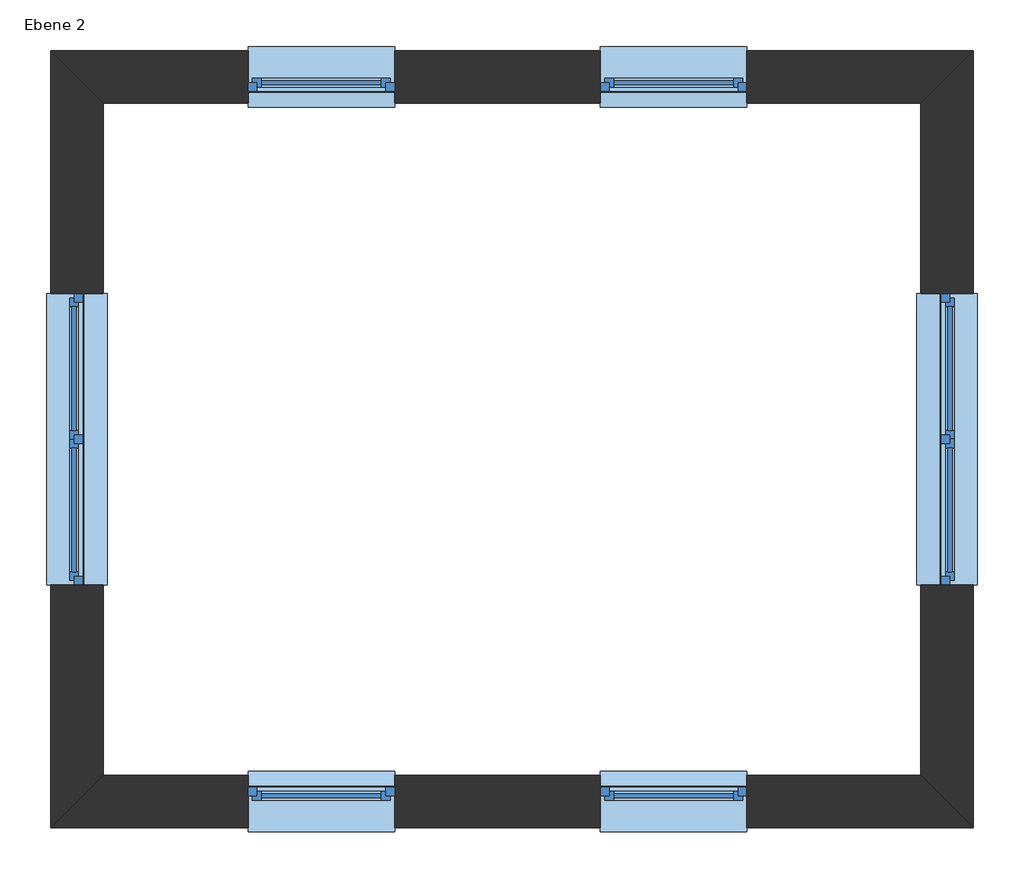
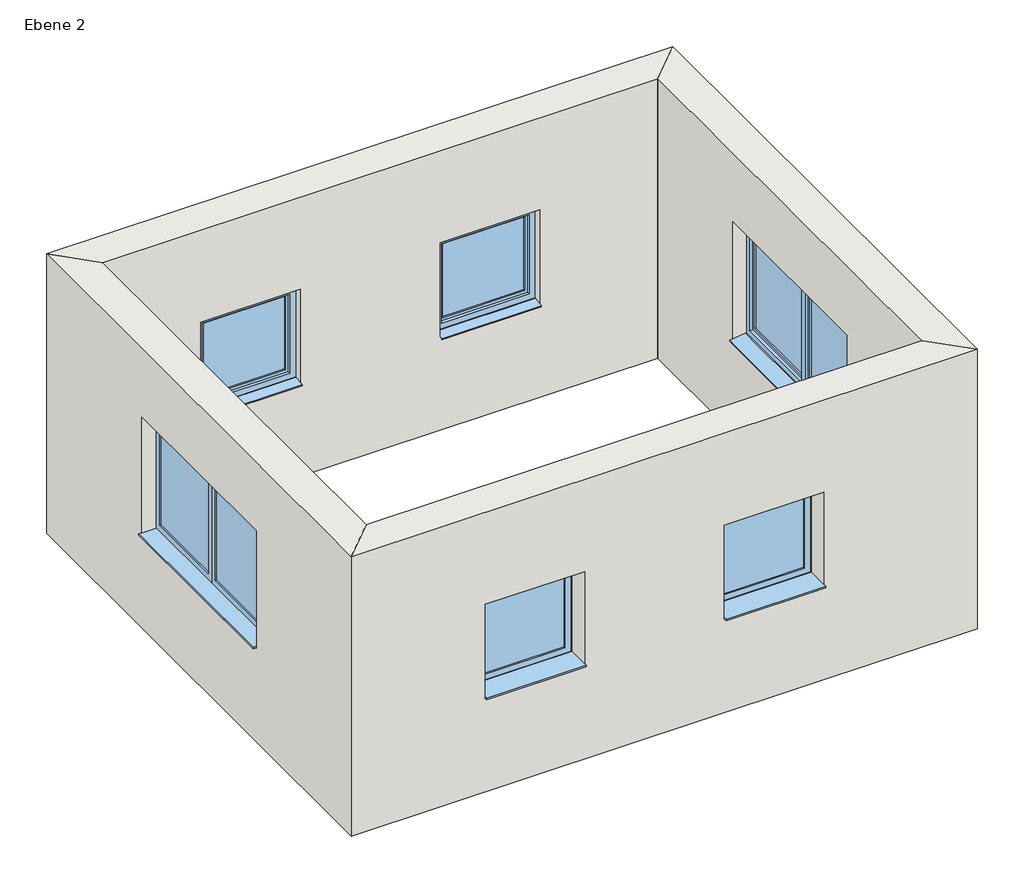
# One storey: 6 windows, 4 walls.
"""IFC4 building model written with IfcOpenShell, lengths in millimetres."""

import ifcopenshell
import ifcopenshell.guid

model = None  # the IFC model being written
_history = None  # IfcOwnerHistory: only IFC2X3 demands one
_inside = {}  # id of a spatial element -> (the spatial element, [elements in it])
_under = {}  # id of a project, library or spatial element -> (it, [spatial elements below it])
_declared = {}  # id of a project -> (the project, [libraries it declares])
_typed = {}  # id of a type object -> (the type object, [elements of that type])
_made_of = {}  # id of a material, layer set ... -> (it, [elements and type objects made of it])


def new_model(schema):
    """Start an empty IFC model of exactly this schema.

    Asked for "IFC4X3", IfcOpenShell would pick the latest addendum, in which some entities
    have other attributes; the version numbers below select the first issue.
    IFC2X3 requires an IfcOwnerHistory on every rooted entity: one is made here for all.
    """
    global model, _history
    if schema == "IFC4X3":
        model = ifcopenshell.file(schema_version=(4, 3, 0, 0))
    else:
        model = ifcopenshell.file(schema=schema)
    _inside.clear()
    _under.clear()
    _declared.clear()
    _typed.clear()
    _made_of.clear()
    _history = None
    if model.schema == "IFC2X3":
        org = make("IfcOrganization", Name="unknown")
        user = make(
            "IfcPersonAndOrganization",
            ThePerson=make("IfcPerson", FamilyName="unknown"),
            TheOrganization=org,
        )
        app = make(
            "IfcApplication",
            ApplicationDeveloper=org,
            Version="unknown",
            ApplicationFullName="unknown",
            ApplicationIdentifier="unknown",
        )
        _history = make(
            "IfcOwnerHistory",
            OwningUser=user,
            OwningApplication=app,
            ChangeAction="ADDED",
            CreationDate=0,
        )
    return model


def make(cls, **values):
    """One entity of the class cls with the attributes given. An attribute that is None is left unset."""
    return model.create_entity(
        cls, **{name: value for name, value in values.items() if value is not None}
    )


def rooted(cls, **values):
    """An entity with a GlobalId (a new one), such as an element, a storey or a relation."""
    return make(cls, GlobalId=ifcopenshell.guid.new(), OwnerHistory=_history, **values)


def si_unit(unit_type, name, prefix=None):
    """IfcSIUnit, for example si_unit("LENGTHUNIT", "METRE", prefix="MILLI")."""
    return make("IfcSIUnit", UnitType=unit_type, Prefix=prefix, Name=name)


def assignment(units):
    """IfcUnitAssignment: the units of a project."""
    return None if units is None else make("IfcUnitAssignment", Units=units)


def point(xyz):
    """IfcCartesianPoint."""
    return None if xyz is None else make("IfcCartesianPoint", Coordinates=xyz)


def direction(xyz):
    """IfcDirection."""
    return None if xyz is None else make("IfcDirection", DirectionRatios=xyz)


def frame(location, z_axis=None, x_axis=None):
    """IfcAxis2Placement3D, a coordinate frame: its origin and axes. An axis left out is left unset."""
    return make(
        "IfcAxis2Placement3D",
        Location=point(location),
        Axis=direction(z_axis),
        RefDirection=direction(x_axis),
    )


def origin():
    """The frame at (0, 0, 0) with its axes left unset."""
    return frame((0.0, 0.0, 0.0))


def place(relative_to, where):
    """IfcLocalPlacement: puts the frame where relative to a parent placement (None: the world)."""
    return make(
        "IfcLocalPlacement", PlacementRelTo=relative_to, RelativePlacement=where
    )


def context(
    kind, dimensions, precision=None, world=None, true_north=None, identifier=None
):
    """IfcGeometricRepresentationContext, for example the 3D "Model" context."""
    return make(
        "IfcGeometricRepresentationContext",
        ContextIdentifier=identifier,
        ContextType=kind,
        CoordinateSpaceDimension=dimensions,
        Precision=precision,
        WorldCoordinateSystem=world,
        TrueNorth=true_north,
    )


def project(units=None, contexts=None):
    """IfcProject with its units and contexts."""
    return rooted(
        "IfcProject",
        Name="project",
        RepresentationContexts=contexts,
        UnitsInContext=assignment(units),
    )


def spatial(cls, under=None, at=None, **own):
    """A site, building, storey or space (cls), placed at a placement, below another one or the project."""
    s = rooted(cls, ObjectPlacement=at, **own)
    if under is not None:
        _under.setdefault(under.id(), (under, []))[1].append(s)
    return s


def polyline(points):
    """IfcPolyline through the points."""
    return make("IfcPolyline", Points=[point(p) for p in points])


def outline(outer, holes=None, kind="AREA"):
    """IfcArbitraryClosedProfileDef: a profile drawn as a closed curve; with holes, ...WithVoids."""
    if holes is None:
        return make("IfcArbitraryClosedProfileDef", ProfileType=kind, OuterCurve=outer)
    return make(
        "IfcArbitraryProfileDefWithVoids",
        ProfileType=kind,
        OuterCurve=outer,
        InnerCurves=holes,
    )


def extrude(swept, where, along, depth):
    """IfcExtrudedAreaSolid: the profile swept, set in the frame where, extruded along a direction by depth."""
    return make(
        "IfcExtrudedAreaSolid",
        SweptArea=swept,
        Position=where,
        ExtrudedDirection=direction(along),
        Depth=depth,
    )


def faces_of(points, faces, orient=None, outer=None):
    """IfcFace entities. A face is a list of loops; a loop is a list of indices into points, from 0.

    orient and outer hold one flag for each loop. By default every Orientation is true, the
    first loop of a face is its IfcFaceOuterBound and the others are IfcFaceBound.
    """
    made = []
    for i, loops in enumerate(faces):
        bounds = []
        for j, loop in enumerate(loops):
            is_outer = j == 0 if outer is None else outer[i][j]
            bounds.append(
                make(
                    "IfcFaceOuterBound" if is_outer else "IfcFaceBound",
                    Bound=make("IfcPolyLoop", Polygon=[points[k] for k in loop]),
                    Orientation=True if orient is None else orient[i][j],
                )
            )
        made.append(make("IfcFace", Bounds=bounds))
    return made


def faceted_brep(points, faces, orient=None, outer=None, voids=None):
    """IfcFacetedBrep: a solid bounded by flat faces; with voids (closed shells), ...WithVoids."""
    shared = [point(p) for p in points]
    hull = make("IfcClosedShell", CfsFaces=faces_of(shared, faces, orient, outer))
    if voids is None:
        return make("IfcFacetedBrep", Outer=hull)
    return make(
        "IfcFacetedBrepWithVoids",
        Outer=hull,
        Voids=[
            make(cls, CfsFaces=faces_of(shared, fs, o, b)) for cls, fs, o, b in voids
        ],
    )


def shape(context_of_items, identifier, shape_type, items):
    """IfcShapeRepresentation: the items that make up one representation, for example the "Body"."""
    return make(
        "IfcShapeRepresentation",
        ContextOfItems=context_of_items,
        RepresentationIdentifier=identifier,
        RepresentationType=shape_type,
        Items=items,
    )


def source(mapping_origin, context_of_items, identifier, shape_type, items):
    """IfcRepresentationMap: a shape defined once, which mapped items show again and again."""
    return make(
        "IfcRepresentationMap",
        MappingOrigin=mapping_origin,
        MappedRepresentation=shape(context_of_items, identifier, shape_type, items),
    )


def transform(
    local_origin,
    x_axis=None,
    y_axis=None,
    z_axis=None,
    scale=None,
    scale2=None,
    scale3=None,
    uniform=True,
):
    """IfcCartesianTransformationOperator3D, or its non-uniform kind. x_axis, y_axis, z_axis: its Axis1, 2, 3."""
    if uniform:
        return make(
            "IfcCartesianTransformationOperator3D",
            Axis1=direction(x_axis),
            Axis2=direction(y_axis),
            LocalOrigin=point(local_origin),
            Scale=scale,
            Axis3=direction(z_axis),
        )
    return make(
        "IfcCartesianTransformationOperator3DnonUniform",
        Axis1=direction(x_axis),
        Axis2=direction(y_axis),
        LocalOrigin=point(local_origin),
        Scale=scale,
        Axis3=direction(z_axis),
        Scale2=scale2,
        Scale3=scale3,
    )


def mapped(mapping_source, mapping_target):
    """IfcMappedItem: shows the shape of a source again, moved by a transform."""
    return make(
        "IfcMappedItem", MappingSource=mapping_source, MappingTarget=mapping_target
    )


def made_of(thing, what):
    """Note that an element or type object is made of a material, layer set ...; save() writes the relation."""
    if what is not None:
        _made_of.setdefault(what.id(), (what, []))[1].append(thing)
    return thing


def element(
    cls,
    number,
    at=None,
    inside=None,
    cuts=None,
    type_object=None,
    material=None,
    context=None,
    identifier="Body",
    shape_type=None,
    held_by="IfcProductDefinitionShape",
    body=None,
    shapes=None,
    **own,
):
    """One element of the class cls, such as IfcWall. Its Tag is "e" and its number.

    at: its placement. inside: the storey or other place that contains it. cuts: it is an
    opening in that element (IfcRelVoidsElement). A single representation is given by context,
    identifier, shape_type and body (its items); several are given by shapes. held_by: the class
    of the entity that holds the representations. save() writes the other relations.
    """
    e = rooted(cls, Tag="e%d" % number, ObjectPlacement=at, **own)
    if body is not None:
        shapes = [shape(context, identifier, shape_type, body)]
    if shapes is not None:
        e.Representation = make(held_by, Representations=shapes)
    if inside is not None:
        _inside.setdefault(inside.id(), (inside, []))[1].append(e)
    if cuts is not None:
        rooted(
            "IfcRelVoidsElement", RelatingBuildingElement=cuts, RelatedOpeningElement=e
        )
    if type_object is not None:
        _typed.setdefault(type_object.id(), (type_object, []))[1].append(e)
    return made_of(e, material)


def aggregate(whole, parts):
    """IfcRelAggregates: a whole, such as a stair, and the parts it consists of."""
    return rooted("IfcRelAggregates", RelatingObject=whole, RelatedObjects=parts)


def save(model, path):
    """Write the relations noted so far, then the file.

    IfcRelAggregates (storeys below a building ...), IfcRelContainedInSpatialStructure (elements
    in a storey), IfcRelDefinesByType, IfcRelAssociatesMaterial and IfcRelDeclares: one each for
    every whole, place, type object, material and project.
    """
    for whole, parts in _under.values():
        aggregate(whole, parts)
    for where, things in _inside.values():
        rooted(
            "IfcRelContainedInSpatialStructure",
            RelatedElements=things,
            RelatingStructure=where,
        )
    for kind, things in _typed.values():
        rooted("IfcRelDefinesByType", RelatedObjects=things, RelatingType=kind)
    for what, things in _made_of.values():
        rooted("IfcRelAssociatesMaterial", RelatedObjects=things, RelatingMaterial=what)
    for by, libraries in _declared.values():
        rooted("IfcRelDeclares", RelatingContext=by, RelatedDefinitions=libraries)
    model.write(path)


def fenster_1_flg_variabel_fenster_1_flg_variabel_3_8a378bad(model_context):
    return source(origin(), model_context, "Body", "SolidModel", [
        extrude(outline(polyline([(2010.0, 505.0), (2010.0, -505.0), (1000.0, -505.0), (1000.0, 505.0), (2010.0, 505.0)]), holes=[polyline([(1930.0, 445.0), (1080.0, 445.0), (1080.0, -445.0), (1930.0, -445.0), (1930.0, 445.0)])]), frame((0.0, 40.0, 0.0), z_axis=(0.0, 1.0, 0.0), x_axis=(0.0, 0.0, 1.0)), (0.0, 0.0, 1.0), 60.0),
        faceted_brep([(475.0, 40.0, 1960.0), (475.0, 10.0, 1960.0), (475.0, 10.0, 1050.0), (475.0, 40.0, 1050.0), (-475.0, 10.0, 1960.0), (-475.0, 10.0, 1050.0), (415.0, 10.0, 1110.0), (-415.0, 10.0, 1110.0), (-415.0, 10.0, 1900.0), (415.0, 10.0, 1900.0), (-475.0, 40.0, 1050.0), (-475.0, 40.0, 1960.0), (445.0, 40.0, 1930.0), (-445.0, 40.0, 1930.0), (-445.0, 40.0, 1080.0), (445.0, 40.0, 1080.0), (445.0, 70.0, 1930.0), (445.0, 70.0, 1080.0), (-445.0, 70.0, 1080.0), (-445.0, 70.0, 1930.0), (415.0, 70.0, 1900.0), (-415.0, 70.0, 1900.0), (-415.0, 70.0, 1110.0), (415.0, 70.0, 1110.0)], [[[0, 1, 2, 3]], [[1, 4, 5, 2], [6, 7, 8, 9]], [[3, 2, 5, 10]], [[3, 10, 11, 0], [12, 13, 14, 15]], [[16, 12, 15, 17]], [[17, 15, 14, 18]], [[17, 18, 19, 16], [20, 21, 22, 23]], [[9, 20, 23, 6]], [[6, 23, 22, 7]], [[10, 5, 4, 11]], [[18, 14, 13, 19]], [[7, 22, 21, 8]], [[11, 4, 1, 0]], [[19, 13, 12, 16]], [[8, 21, 20, 9]]]),
        extrude(outline(polyline([(-505.0, -210.0), (-505.0, 40.0), (505.0, 40.0), (505.0, -210.0), (-505.0, -210.0)])), frame((0.0, 0.0, 1005.0), z_axis=(0.0, 0.0, 1.0), x_axis=(1.0, 0.0, 0.0)), (0.0, 0.0, 1.0), 15.0),
        extrude(outline(polyline([(110.0221543, 1020.0), (210.0, 1000.0), (210.0, 990.0), (208.0, 990.0), (208.0, 998.3604634), (109.8240723, 1018.0), (100.0, 1018.0), (100.0, 1020.0), (110.0221543, 1020.0)])), frame((-505.0, 0.0, 0.0), z_axis=(1.0, 0.0, 0.0), x_axis=(0.0, 1.0, 0.0)), (0.0, 0.0, 1.0), 1010.0),
        extrude(outline(polyline([(415.0, 25.0), (-415.0, 25.0), (-415.0, 55.0), (415.0, 55.0), (415.0, 25.0)])), frame((0.0, 0.0, 1110.0), z_axis=(0.0, 0.0, 1.0), x_axis=(1.0, 0.0, 0.0)), (0.0, 0.0, 1.0), 790.0),
    ])


def fenster_2_flg_variabel_fenster_2_flg_variabel_3_03287464(model_context):
    return source(origin(), model_context, "Body", "SolidModel", [
        extrude(outline(polyline([(60.0, -5.0), (915.0, -5.0), (915.0, -35.0), (60.0, -35.0), (60.0, -5.0)])), frame((0.0, 0.0, 1110.0), z_axis=(0.0, 0.0, 1.0), x_axis=(1.0, 0.0, 0.0)), (0.0, 0.0, 1.0), 1040.0),
        extrude(outline(polyline([(-915.0, -5.0), (-60.0, -5.0), (-60.0, -35.0), (-915.0, -35.0), (-915.0, -5.0)])), frame((0.0, 0.0, 1110.0), z_axis=(0.0, 0.0, 1.0), x_axis=(1.0, 0.0, 0.0)), (0.0, 0.0, 1.0), 1040.0),
        extrude(outline(polyline([(-1005.0, -210.0), (-1005.0, -20.0), (1005.0, -20.0), (1005.0, -210.0), (-1005.0, -210.0)])), frame((0.0, 0.0, 1005.0), z_axis=(0.0, 0.0, 1.0), x_axis=(1.0, 0.0, 0.0)), (0.0, 0.0, 1.0), 15.0),
        extrude(outline(polyline([(50.0221543, 1020.0), (210.0, 1000.0), (210.0, 990.0), (208.0, 990.0), (208.0, 998.3604634), (49.8240723, 1018.0), (40.0, 1018.0), (40.0, 1020.0), (50.0221543, 1020.0)])), frame((-1005.0, 0.0, 0.0), z_axis=(1.0, 0.0, 0.0), x_axis=(0.0, 1.0, 0.0)), (0.0, 0.0, 1.0), 2010.0),
        extrude(outline(polyline([(30.0, -20.0), (-30.0, -20.0), (-30.0, 40.0), (30.0, 40.0), (30.0, -20.0)])), frame((0.0, 0.0, 1080.0), z_axis=(0.0, 0.0, 1.0), x_axis=(1.0, 0.0, 0.0)), (0.0, 0.0, 1.0), 1100.0),
        extrude(outline(polyline([(2260.0, -1005.0), (1000.0, -1005.0), (1000.0, 1005.0), (2260.0, 1005.0), (2260.0, -1005.0)]), holes=[polyline([(2180.0, -945.0), (2180.0, 945.0), (1080.0, 945.0), (1080.0, -945.0), (2180.0, -945.0)])]), frame((0.0, -20.0, 0.0), z_axis=(0.0, 1.0, 0.0), x_axis=(0.0, 0.0, 1.0)), (0.0, 0.0, 1.0), 60.0),
        faceted_brep([(-945.0, -20.0, 1080.0), (-945.0, 10.0, 1080.0), (-30.0, 10.0, 1080.0), (-30.0, -20.0, 1080.0), (-30.0, 10.0, 2180.0), (-30.0, -20.0, 2180.0), (-945.0, 10.0, 2180.0), (-60.0, 10.0, 2150.0), (-915.0, 10.0, 2150.0), (-915.0, 10.0, 1110.0), (-60.0, 10.0, 1110.0), (0.0, -20.0, 1050.0), (-975.0, -20.0, 1050.0), (-975.0, -20.0, 2210.0), (0.0, -20.0, 2210.0), (-945.0, -20.0, 2180.0), (-975.0, -50.0, 1050.0), (0.0, -50.0, 1050.0), (0.0, -50.0, 2210.0), (-975.0, -50.0, 2210.0), (-60.0, -50.0, 1110.0), (-915.0, -50.0, 1110.0), (-915.0, -50.0, 2150.0), (-60.0, -50.0, 2150.0)], [[[0, 1, 2, 3]], [[3, 2, 4, 5]], [[2, 1, 6, 4], [7, 8, 9, 10]], [[11, 12, 13, 14], [5, 15, 0, 3]], [[16, 12, 11, 17]], [[17, 11, 14, 18]], [[18, 19, 16, 17], [20, 21, 22, 23]], [[9, 21, 20, 10]], [[10, 20, 23, 7]], [[15, 6, 1, 0]], [[19, 13, 12, 16]], [[8, 22, 21, 9]], [[5, 4, 6, 15]], [[18, 14, 13, 19]], [[7, 23, 22, 8]]]),
        faceted_brep([(30.0, -20.0, 1080.0), (30.0, 10.0, 1080.0), (945.0, 10.0, 1080.0), (945.0, -20.0, 1080.0), (945.0, 10.0, 2180.0), (945.0, -20.0, 2180.0), (30.0, 10.0, 2180.0), (915.0, 10.0, 2150.0), (60.0, 10.0, 2150.0), (60.0, 10.0, 1110.0), (915.0, 10.0, 1110.0), (975.0, -20.0, 1050.0), (0.0, -20.0, 1050.0), (0.0, -20.0, 2210.0), (975.0, -20.0, 2210.0), (30.0, -20.0, 2180.0), (0.0, -50.0, 1050.0), (975.0, -50.0, 1050.0), (975.0, -50.0, 2210.0), (0.0, -50.0, 2210.0), (915.0, -50.0, 1110.0), (60.0, -50.0, 1110.0), (60.0, -50.0, 2150.0), (915.0, -50.0, 2150.0)], [[[0, 1, 2, 3]], [[3, 2, 4, 5]], [[2, 1, 6, 4], [7, 8, 9, 10]], [[11, 12, 13, 14], [5, 15, 0, 3]], [[16, 12, 11, 17]], [[17, 11, 14, 18]], [[18, 19, 16, 17], [20, 21, 22, 23]], [[9, 21, 20, 10]], [[10, 20, 23, 7]], [[15, 6, 1, 0]], [[19, 13, 12, 16]], [[8, 22, 21, 9]], [[5, 4, 6, 15]], [[18, 14, 13, 19]], [[7, 23, 22, 8]]]),
    ])


model = new_model("IFC4")

# Units and contexts
model_context = context("Model", 3, world=origin())
ifc_project = project(units=[si_unit("LENGTHUNIT", "METRE", prefix="MILLI")], contexts=[model_context])

# Site, building, storey
site = spatial("IfcSite", under=ifc_project)
building = spatial("IfcBuilding", under=site)
storey = spatial("IfcBuildingStorey", under=building, Name="Ebene 2", Elevation=6000.0)

# Walls
placement = place(None, origin())
element("IfcWall", 1, ObjectType="MW 24.0 WD 12.0", at=placement, inside=storey, context=model_context, shape_type="Brep", body=[
    faceted_brep([(-6003.5987005, 5004.2257101, 6000.0), (-363.5987005, 5004.2257101, 6000.0), (-363.5987005, 5004.2257101, 9000.0), (-6003.5987005, 5004.2257101, 9000.0), (-1563.5987005, 5004.2257101, 7000.0), (-2573.5987005, 5004.2257101, 7000.0), (-2573.5987005, 5004.2257101, 8010.0), (-1563.5987005, 5004.2257101, 8010.0), (-3993.5987005, 5004.2257101, 7000.0), (-5003.5987005, 5004.2257101, 7000.0), (-5003.5987005, 5004.2257101, 8010.0), (-3993.5987005, 5004.2257101, 8010.0), (-6363.5987005, 5364.2257101, 6000.0), (-6363.5987005, 5364.2257101, 9000.0), (-3.5987005, 5364.2257101, 9000.0), (-3.5987005, 5364.2257101, 6000.0), (-1563.5987005, 5364.2257101, 7000.0), (-1563.5987005, 5364.2257101, 8010.0), (-2573.5987005, 5364.2257101, 8010.0), (-2573.5987005, 5364.2257101, 7000.0), (-3993.5987005, 5364.2257101, 7000.0), (-3993.5987005, 5364.2257101, 8010.0), (-5003.5987005, 5364.2257101, 8010.0), (-5003.5987005, 5364.2257101, 7000.0)], [[[0, 1, 2, 3], [4, 5, 6, 7], [8, 9, 10, 11]], [[12, 13, 14, 15], [16, 17, 18, 19], [20, 21, 22, 23]], [[1, 0, 12, 15]], [[3, 2, 14, 13]], [[2, 1, 15, 14]], [[0, 3, 13, 12]], [[17, 16, 4, 7]], [[18, 17, 7, 6]], [[19, 18, 6, 5]], [[16, 19, 5, 4]], [[21, 20, 8, 11]], [[22, 21, 11, 10]], [[23, 22, 10, 9]], [[20, 23, 9, 8]]]),
])
element("IfcWall", 2, ObjectType="MW 24.0 WD 12.0", at=placement, inside=storey, context=model_context, shape_type="Brep", body=[
    faceted_brep([(-363.5987005, 5004.2257101, 6000.0), (-363.5987005, 364.2257101, 6000.0), (-363.5987005, 364.2257101, 9000.0), (-363.5987005, 5004.2257101, 9000.0), (-363.5987005, 1679.2257101, 7000.0), (-363.5987005, 3689.2257101, 7000.0), (-363.5987005, 3689.2257101, 8260.0), (-363.5987005, 1679.2257101, 8260.0), (-3.5987005, 5364.2257101, 6000.0), (-3.5987005, 5364.2257101, 9000.0), (-3.5987005, 4.2257101, 9000.0), (-3.5987005, 4.2257101, 6000.0), (-3.5987005, 1679.2257101, 7000.0), (-3.5987005, 1679.2257101, 8260.0), (-3.5987005, 3689.2257101, 8260.0), (-3.5987005, 3689.2257101, 7000.0)], [[[0, 1, 2, 3], [4, 5, 6, 7]], [[8, 9, 10, 11], [12, 13, 14, 15]], [[1, 0, 8, 11]], [[3, 2, 10, 9]], [[0, 3, 9, 8]], [[2, 1, 11, 10]], [[13, 12, 4, 7]], [[14, 13, 7, 6]], [[15, 14, 6, 5]], [[12, 15, 5, 4]]]),
])
element("IfcWall", 3, ObjectType="MW 24.0 WD 12.0", at=placement, inside=storey, context=model_context, shape_type="Brep", body=[
    faceted_brep([(-363.5987005, 364.2257101, 6000.0), (-6003.5987005, 364.2257101, 6000.0), (-6003.5987005, 364.2257101, 9000.0), (-363.5987005, 364.2257101, 9000.0), (-2573.5987005, 364.2257101, 7000.0), (-1563.5987005, 364.2257101, 7000.0), (-1563.5987005, 364.2257101, 8010.0), (-2573.5987005, 364.2257101, 8010.0), (-5003.5987005, 364.2257101, 7000.0), (-3993.5987005, 364.2257101, 7000.0), (-3993.5987005, 364.2257101, 8010.0), (-5003.5987005, 364.2257101, 8010.0), (-3.5987005, 4.2257101, 6000.0), (-3.5987005, 4.2257101, 9000.0), (-6363.5987005, 4.2257101, 9000.0), (-6363.5987005, 4.2257101, 6000.0), (-2573.5987005, 4.2257101, 7000.0), (-2573.5987005, 4.2257101, 8010.0), (-1563.5987005, 4.2257101, 8010.0), (-1563.5987005, 4.2257101, 7000.0), (-5003.5987005, 4.2257101, 7000.0), (-5003.5987005, 4.2257101, 8010.0), (-3993.5987005, 4.2257101, 8010.0), (-3993.5987005, 4.2257101, 7000.0)], [[[0, 1, 2, 3], [4, 5, 6, 7], [8, 9, 10, 11]], [[12, 13, 14, 15], [16, 17, 18, 19], [20, 21, 22, 23]], [[1, 0, 12, 15]], [[3, 2, 14, 13]], [[0, 3, 13, 12]], [[2, 1, 15, 14]], [[17, 16, 4, 7]], [[18, 17, 7, 6]], [[19, 18, 6, 5]], [[16, 19, 5, 4]], [[21, 20, 8, 11]], [[22, 21, 11, 10]], [[23, 22, 10, 9]], [[20, 23, 9, 8]]]),
])
element("IfcWall", 4, ObjectType="MW 24.0 WD 12.0", at=placement, inside=storey, context=model_context, shape_type="Brep", body=[
    faceted_brep([(-6003.5987005, 364.2257101, 6000.0), (-6003.5987005, 5004.2257101, 6000.0), (-6003.5987005, 5004.2257101, 9000.0), (-6003.5987005, 364.2257101, 9000.0), (-6003.5987005, 3689.2257101, 7000.0), (-6003.5987005, 1679.2257101, 7000.0), (-6003.5987005, 1679.2257101, 8260.0), (-6003.5987005, 3689.2257101, 8260.0), (-6363.5987005, 4.2257101, 6000.0), (-6363.5987005, 4.2257101, 9000.0), (-6363.5987005, 5364.2257101, 9000.0), (-6363.5987005, 5364.2257101, 6000.0), (-6363.5987005, 3689.2257101, 7000.0), (-6363.5987005, 3689.2257101, 8260.0), (-6363.5987005, 1679.2257101, 8260.0), (-6363.5987005, 1679.2257101, 7000.0)], [[[0, 1, 2, 3], [4, 5, 6, 7]], [[8, 9, 10, 11], [12, 13, 14, 15]], [[1, 0, 8, 11]], [[3, 2, 10, 9]], [[2, 1, 11, 10]], [[0, 3, 9, 8]], [[13, 12, 4, 7]], [[14, 13, 7, 6]], [[15, 14, 6, 5]], [[12, 15, 5, 4]]]),
])

# Windows
fenster_1_flg_variabel_fenster_1_flg_variabel_3_shape = fenster_1_flg_variabel_fenster_1_flg_variabel_3_8a378bad(model_context)
element("IfcWindow", 5, ObjectType="Fenster 1-flg - Variabel : Fenster 1-flg - Variabel 3", at=placement, inside=storey, context=model_context, shape_type="MappedRepresentation", body=[
    mapped(fenster_1_flg_variabel_fenster_1_flg_variabel_3_shape, transform((-2068.5987005, 184.2257101, 6000.0), x_axis=(1.0, 0.0, 0.0), y_axis=(0.0, 1.0, 0.0), z_axis=(0.0, 0.0, 1.0))),
])
element("IfcWindow", 6, ObjectType="Fenster 1-flg - Variabel : Fenster 1-flg - Variabel 3", at=placement, inside=storey, context=model_context, shape_type="MappedRepresentation", body=[
    mapped(fenster_1_flg_variabel_fenster_1_flg_variabel_3_shape, transform((-4498.5987005, 184.2257101, 6000.0), x_axis=(1.0, 0.0, 0.0), y_axis=(0.0, 1.0, 0.0), z_axis=(0.0, 0.0, 1.0))),
])
element("IfcWindow", 7, ObjectType="Fenster 1-flg - Variabel : Fenster 1-flg - Variabel 3", at=placement, inside=storey, context=model_context, shape_type="MappedRepresentation", body=[
    mapped(fenster_1_flg_variabel_fenster_1_flg_variabel_3_shape, transform((-2068.5987005, 5184.2257101, 6000.0), x_axis=(-1.0, 0.0, 0.0), y_axis=(0.0, -1.0, 0.0), z_axis=(0.0, 0.0, 1.0))),
])
element("IfcWindow", 8, ObjectType="Fenster 1-flg - Variabel : Fenster 1-flg - Variabel 3", at=placement, inside=storey, context=model_context, shape_type="MappedRepresentation", body=[
    mapped(fenster_1_flg_variabel_fenster_1_flg_variabel_3_shape, transform((-4498.5987005, 5184.2257101, 6000.0), x_axis=(-1.0, 0.0, 0.0), y_axis=(0.0, -1.0, 0.0), z_axis=(0.0, 0.0, 1.0))),
])
fenster_2_flg_variabel_fenster_2_flg_variabel_3_shape = fenster_2_flg_variabel_fenster_2_flg_variabel_3_03287464(model_context)
element("IfcWindow", 9, ObjectType="Fenster 2-flg - Variabel : Fenster 2-flg - Variabel 3", at=placement, inside=storey, context=model_context, shape_type="MappedRepresentation", body=[
    mapped(fenster_2_flg_variabel_fenster_2_flg_variabel_3_shape, transform((-183.5987005, 2684.2257101, 6000.0), x_axis=(0.0, 1.0, 0.0), y_axis=(-1.0, 0.0, 0.0), z_axis=(0.0, 0.0, 1.0))),
])
element("IfcWindow", 10, ObjectType="Fenster 2-flg - Variabel : Fenster 2-flg - Variabel 3", at=placement, inside=storey, context=model_context, shape_type="MappedRepresentation", body=[
    mapped(fenster_2_flg_variabel_fenster_2_flg_variabel_3_shape, transform((-6183.5987005, 2684.2257101, 6000.0), x_axis=(0.0, -1.0, 0.0), y_axis=(1.0, 0.0, 0.0), z_axis=(0.0, 0.0, 1.0))),
])

save(model, "model.ifc")

# Revit data of these elements
# Type "MW 24.0 WD 12.0"
#   Type Comments = "Mehrschaliges Mauerwerk"
#   Description = "Mauerwerk 24.0 cm, Wärmedämmung 12.0 cm"
#   Layers, outside or top first: 0.120 m "Wärmedämmung - hart" (function 3); 0.240 m "Mauerwerk - Ziegel, verputzt" (function 1)
# Type "Fenster 1-flg - Variabel : Fenster 1-flg - Variabel 3"
#   Type Mark = "52"
#   Operation = "SinglePanel"
#   Construction Type Id = "GSP4R"
#   Keynote = "16.05.01"
#   Analytic Construction = "1/8 Zoll Pilkington-Verglasung einfach"
#   Cost = 78.2
#   Visual Light Transmittance = 0.9
#   Höhe oberer  Rahmen = 0.080 m
#   Solar Heat Gain Coefficient = 0.86
#   Tiefe Flügel = 0.060 m
#   Rough Width [instance default] = 1.010 m
#   Rough Height [instance default] = 1.010 m
#   Rahmenhöhe unten = 0.080 m
#   Heat Transfer Coefficient (U) = 6.7069 W/(m²·K)
#   Rahmentiefe = 0.060 m
#   Rahmenbreite = 0.060 m
#   Height [instance default] = 1.010 m
#   Flügelbreite = 0.060 m
#   Einbautiefe (von außen) [instance default] = 0.080 m
#   Width [instance default] = 1.010 m
#   Define Thermal Properties by = 1
#   Öffnungsrichtung oben [instance default] = yes
#   Öffnungsrichtung in Draufsicht anzeigen [instance default] = no
#   Klappflügel [instance default] = no
#   Drehflügel 1 [instance default] = yes
#   Fensterflügel [instance default] = none
#   Innere Fensterbank [instance default] = none
#   Glas [instance default] = none
#   Bild [instance default] = none
#   Äußere Fensterbank [instance default] = none
#   Wall Closure = (empty or 0)
# Type "Fenster 2-flg - Variabel : Fenster 2-flg - Variabel 3"
#   Type Mark = "53"
#   Operation = "DoublePanelVertical"
#   Construction Type Id = "GSP4R"
#   Keynote = "16.05.01"
#   Analytic Construction = "1/8 Zoll Pilkington-Verglasung einfach"
#   Cost = 130.98
#   Visual Light Transmittance = 0.9
#   Solar Heat Gain Coefficient = 0.78
#   Rough Width [instance default] = 2.010 m
#   Rough Height [instance default] = 1.260 m
#   Heat Transfer Coefficient (U) = 3.6886 W/(m²·K)
#   Rahmentiefe = 0.060 m
#   Rahmenhöhe unten = 0.080 m
#   Höhe oberer  Rahmen = 0.080 m
#   Rahmenbreite = 0.060 m
#   Height [instance default] = 1.260 m
#   Tiefe Flügel = 0.060 m
#   Flügelbreite = 0.060 m
#   Einbautiefe (von außen) [instance default] = 0.140 m
#   Width [instance default] = 2.010 m
#   Define Thermal Properties by = 1
#   Öffnungsrichtung oben [instance default] = yes
#   Öffnungsrichtung in Draufsicht anzeigen [instance default] = no
#   Drehflügel 1 [instance default] = yes
#   Bild [instance default] = none
#   Glas [instance default] = none
#   Fensterflügel [instance default] = none
#   Äußere Fensterbank [instance default] = none
#   Innere Fensterbank [instance default] = none
#   Wall Closure = (empty or 0)
# Elements 1, 2, 3, 4 (IfcWall, "MW 24.0 WD 12.0")
#   Comments = ""
#   Top Offset = 0.000 m
#   Base Offset = 0.000 m
#   Unconnected Height = 3.000 m
#   wall height = 3.000 m
#   Phase Created = Phase 1
#   Base Constraint = Ebene 2
#   Materials on its faces: "Vorgabe - Wand", "Mauerwerk - Ziegel, verputzt", "Wärmedämmung - hart"
# Element 5 (IfcWindow, "Fenster 1-flg - Variabel : Fenster 1-flg - Variabel 3")
#   Mark = "10"
#   Rough Height = 1.010 m
#   Rough Width = 1.010 m
#   Height = 1.010 m
#   Einbautiefe (von außen) = 0.080 m
#   Width = 1.010 m
#   Öffnungsrichtung oben = yes
#   Öffnungsrichtung in Draufsicht anzeigen = no
#   Klappflügel = no
#   Drehflügel 1 = yes
#   Äußere Fensterbank = none
#   Innere Fensterbank = none
#   Glas = none
#   Fensterflügel = none
#   Bild = none
#   Phase Created = Phase 1
#   Materials on its faces: "Kunststoff - Weiß", "Holz - Birke", "Glas"
# Element 6 (IfcWindow, "Fenster 1-flg - Variabel : Fenster 1-flg - Variabel 3")
#   Mark = "11"
#   Rough Height = 1.010 m
#   Rough Width = 1.010 m
#   Height = 1.010 m
#   Einbautiefe (von außen) = 0.080 m
#   Width = 1.010 m
#   Öffnungsrichtung oben = yes
#   Öffnungsrichtung in Draufsicht anzeigen = no
#   Klappflügel = no
#   Drehflügel 1 = yes
#   Äußere Fensterbank = none
#   Innere Fensterbank = none
#   Glas = none
#   Fensterflügel = none
#   Bild = none
#   Phase Created = Phase 1
#   Materials on its faces: "Kunststoff - Weiß", "Holz - Birke", "Glas"
# Element 7 (IfcWindow, "Fenster 1-flg - Variabel : Fenster 1-flg - Variabel 3")
#   Mark = "12"
#   Rough Height = 1.010 m
#   Rough Width = 1.010 m
#   Height = 1.010 m
#   Einbautiefe (von außen) = 0.080 m
#   Width = 1.010 m
#   Öffnungsrichtung oben = yes
#   Öffnungsrichtung in Draufsicht anzeigen = no
#   Klappflügel = no
#   Drehflügel 1 = yes
#   Äußere Fensterbank = none
#   Innere Fensterbank = none
#   Glas = none
#   Fensterflügel = none
#   Bild = none
#   Phase Created = Phase 1
#   Materials on its faces: "Kunststoff - Weiß", "Holz - Birke", "Glas"
# Element 8 (IfcWindow, "Fenster 1-flg - Variabel : Fenster 1-flg - Variabel 3")
#   Mark = "13"
#   Rough Height = 1.010 m
#   Rough Width = 1.010 m
#   Height = 1.010 m
#   Einbautiefe (von außen) = 0.080 m
#   Width = 1.010 m
#   Öffnungsrichtung oben = yes
#   Öffnungsrichtung in Draufsicht anzeigen = no
#   Klappflügel = no
#   Drehflügel 1 = yes
#   Äußere Fensterbank = none
#   Innere Fensterbank = none
#   Glas = none
#   Fensterflügel = none
#   Bild = none
#   Phase Created = Phase 1
#   Materials on its faces: "Kunststoff - Weiß", "Holz - Birke", "Glas"
# Element 9 (IfcWindow, "Fenster 2-flg - Variabel : Fenster 2-flg - Variabel 3")
#   Mark = "14"
#   Rough Height = 1.260 m
#   Rough Width = 2.010 m
#   Height = 1.260 m
#   Einbautiefe (von außen) = 0.140 m
#   Width = 2.010 m
#   Öffnungsrichtung oben = yes
#   Öffnungsrichtung in Draufsicht anzeigen = no
#   Drehflügel 1 = yes
#   Äußere Fensterbank = none
#   Innere Fensterbank = none
#   Glas = none
#   Fensterflügel = none
#   Bild = none
#   Phase Created = Phase 1
#   Materials on its faces: "Kunststoff - Weiß", "Glas", "Holz - Birke"
# Element 10 (IfcWindow, "Fenster 2-flg - Variabel : Fenster 2-flg - Variabel 3")
#   Mark = "15"
#   Rough Height = 1.260 m
#   Rough Width = 2.010 m
#   Height = 1.260 m
#   Einbautiefe (von außen) = 0.140 m
#   Width = 2.010 m
#   Öffnungsrichtung oben = yes
#   Öffnungsrichtung in Draufsicht anzeigen = no
#   Drehflügel 1 = yes
#   Äußere Fensterbank = none
#   Innere Fensterbank = none
#   Glas = none
#   Fensterflügel = none
#   Bild = none
#   Phase Created = Phase 1
#   Materials on its faces: "Kunststoff - Weiß", "Glas", "Holz - Birke"
# Materials
#   "Wärmedämmung - hart": class "Stuck", colour RGB 255 255 255, transparency 0, Description = "Äußere Oberfläche", Cost = 0
#   "Mauerwerk - Ziegel, verputzt": class "Stuck", colour RGB 247 247 247, transparency 0, Cost = 0
#   "Vorgabe - Wand": class "Stuck", colour RGB 128 128 128, transparency 0, Description = "Äußere Oberfläche", Cost = 0
#   "Kunststoff - Weiß": class "Kunststoff", colour RGB 249 249 249, transparency 0, Cost = 0
#   "Holz - Birke": class "Holz", colour RGB 213 164 103, transparency 0, Cost = 0
#   "Glas": class "Glas", colour RGB 0 0 255, transparency 0.75, Comments = "Render-Darstellung nicht aktualisiert ", Cost = 0
